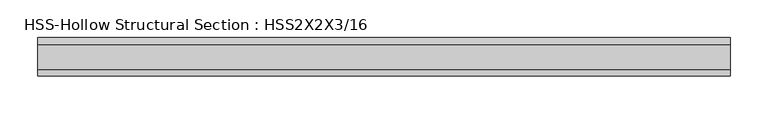
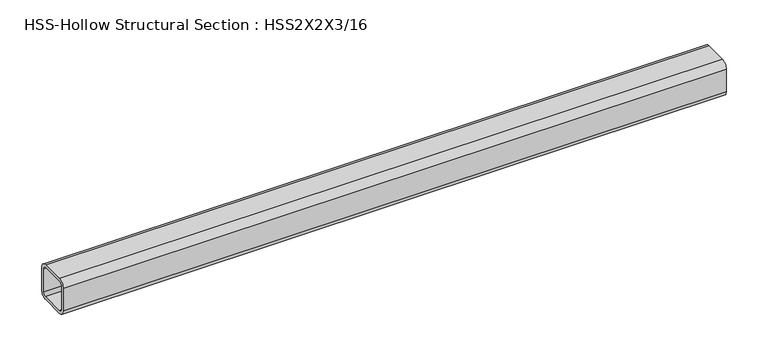
"""IFC4 building model written with IfcOpenShell, lengths in millimetres: beam geometry, HSS-Hollow Structural Section : HSS2X2X3/16."""

from ifc_helpers import new_model, si_unit, point, frame, frame_2d, origin, place, context, project, spatial, polyline, circle_curve, trimmed, segment, composite_curve, outline, extrude, source, transform, mapped, element, save


def hss_hollow_structural_section_hss2x2x3_16_b0a53acd(model_context):
    return source(origin(), model_context, "Body", "SweptSolid", [
        extrude(outline(composite_curve([segment(polyline([(25.4, 16.5608), (25.4, -16.5608)]), True, "CONTINUOUS"), segment(trimmed(circle_curve(frame_2d((16.5608, -16.5608)), 8.8392), [point((25.4, -16.5608))], [point((16.5608, -25.4))], False, "CARTESIAN"), True, "CONTINUOUS"), segment(polyline([(16.5608, -25.4), (-16.5608, -25.4)]), True, "CONTINUOUS"), segment(trimmed(circle_curve(frame_2d((-16.5608, -16.5608)), 8.8392), [point((-16.5608, -25.4))], [point((-25.4, -16.5608))], False, "CARTESIAN"), True, "CONTINUOUS"), segment(polyline([(-25.4, -16.5608), (-25.4, 16.5608)]), True, "CONTINUOUS"), segment(trimmed(circle_curve(frame_2d((-16.5608, 16.5608)), 8.8392), [point((-25.4, 16.5608))], [point((-16.5608, 25.4))], False, "CARTESIAN"), True, "CONTINUOUS"), segment(polyline([(-16.5608, 25.4), (16.5608, 25.4)]), True, "CONTINUOUS"), segment(trimmed(circle_curve(frame_2d((16.5608, 16.5608)), 8.8392), [point((16.5608, 25.4))], [point((25.4, 16.5608))], False, "CARTESIAN"), True, "CONTINUOUS")], self_intersect=False), holes=[composite_curve([segment(trimmed(circle_curve(frame_2d((-16.5608, 16.5608)), 4.4196), [point((-16.5608, 20.9804))], [point((-20.9804, 16.5608))], True, "CARTESIAN"), True, "CONTINUOUS"), segment(polyline([(-20.9804, 16.5608), (-20.9804, -16.5608)]), True, "CONTINUOUS"), segment(trimmed(circle_curve(frame_2d((-16.5608, -16.5608)), 4.4196), [point((-20.9804, -16.5608))], [point((-16.5608, -20.9804))], True, "CARTESIAN"), True, "CONTINUOUS"), segment(polyline([(-16.5608, -20.9804), (16.5608, -20.9804)]), True, "CONTINUOUS"), segment(trimmed(circle_curve(frame_2d((16.5608, -16.5608)), 4.4196), [point((16.5608, -20.9804))], [point((20.9804, -16.5608))], True, "CARTESIAN"), True, "CONTINUOUS"), segment(polyline([(20.9804, -16.5608), (20.9804, 16.5608)]), True, "CONTINUOUS"), segment(trimmed(circle_curve(frame_2d((16.5608, 16.5608)), 4.4196), [point((20.9804, 16.5608))], [point((16.5608, 20.9804))], True, "CARTESIAN"), True, "CONTINUOUS"), segment(polyline([(16.5608, 20.9804), (-16.5608, 20.9804)]), True, "CONTINUOUS")], self_intersect=False)]), frame((8547.89375, 0.0, 0.0), z_axis=(1.0, 0.0, 0.0), x_axis=(0.0, 1.0, 0.0)), (0.0, 0.0, 1.0), 914.4),
    ])


if __name__ == "__main__":
    model = new_model("IFC4")
    model_context = context("Model", 3, world=origin())
    ifc_project = project(units=[si_unit("LENGTHUNIT", "METRE", prefix="MILLI")], contexts=[model_context])
    site = spatial("IfcSite", under=ifc_project)
    building = spatial("IfcBuilding", under=site)
    placement = place(None, origin())
    hss_hollow_structural_section_hss2x2x3_16_shape = hss_hollow_structural_section_hss2x2x3_16_b0a53acd(model_context)
    element("IfcBeam", 1, ObjectType="HSS-Hollow Structural Section : HSS2X2X3/16", at=placement, inside=building, context=model_context, shape_type="MappedRepresentation", body=[
        mapped(hss_hollow_structural_section_hss2x2x3_16_shape, transform((0.0, 0.0, 0.0), x_axis=(1.0, 0.0, 0.0), y_axis=(0.0, 1.0, 0.0), z_axis=(0.0, 0.0, 1.0))),
    ])
    save(model, "model.ifc")

# Revit data of these elements
# Type "HSS-Hollow Structural Section : HSS2X2X3/16"
#   Keynote = "M05121300.04"
#   Assembly Code = "B10"
#   Shape = "Square"
#   W = 4.3
#   Ht = 0' - 2"
#   Length [instance default] = 5' - 0"
#   b = 0' - 2"
#   kr = 0' - 0.348"
#   t = 0' - 0.174"
#   A = 0.00826389 SF
#   Structural Material [instance default] = Steel ASTM A500, Grade B, Rectangular and Square
# Element 1 (IfcBeam, "HSS-Hollow Structural Section : HSS2X2X3/16")
#   Materials on its faces: "Steel ASTM A500, Grade B, Rectangular and Square"
# Materials
#   "Steel ASTM A500, Grade B, Rectangular and Square": class "Metal", colour RGB 199 199 199, transparency 0, Description = "Carbon steel", Cost = 0
